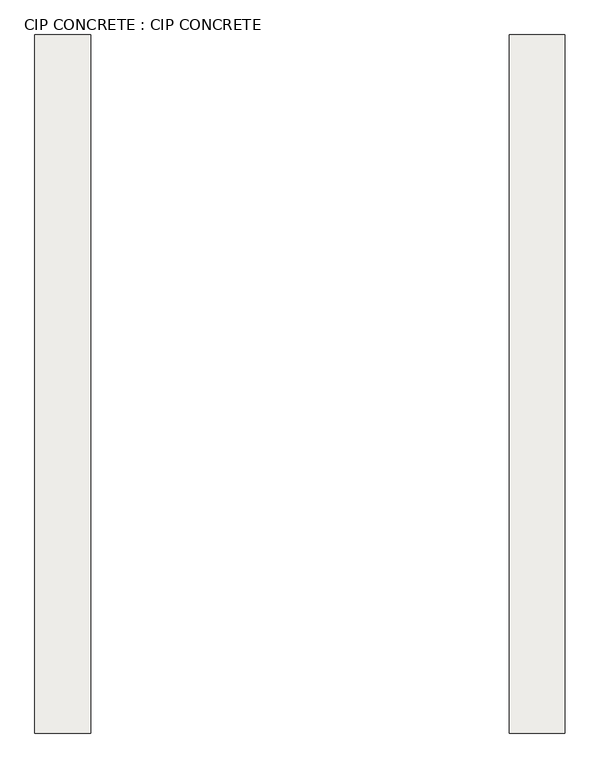
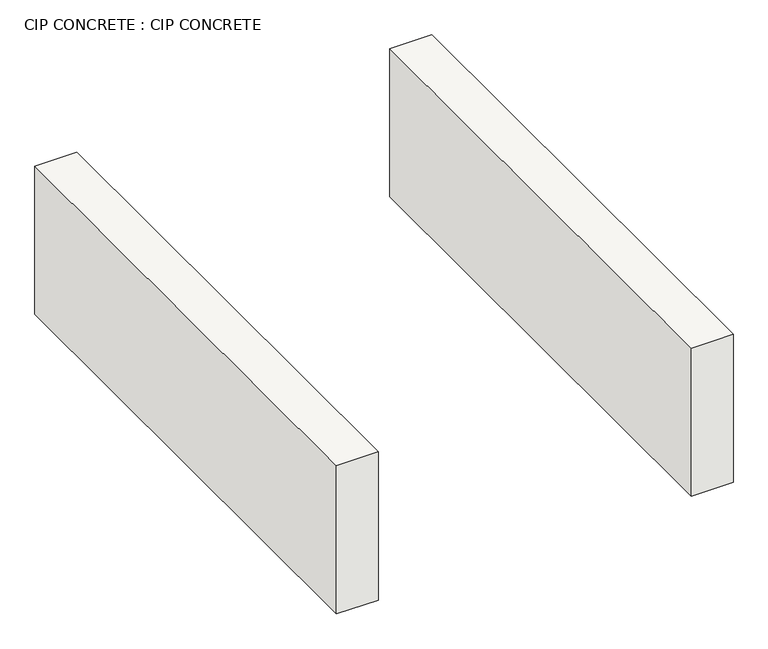
"""IFC4 building model written with IfcOpenShell, lengths in millimetres: slab geometry, CIP CONCRETE : CIP CONCRETE."""

from ifc_helpers import new_model, si_unit, frame, origin, place, context, project, spatial, polyline, outline, extrude, source, transform, mapped, element, save


def cip_concrete_cip_concrete_0247726a(model_context):
    return source(origin(), model_context, "Body", "SweptSolid", [
        extrude(outline(polyline([(14020.0, 38279.5208589), (14020.0, 33279.5208589), (13620.0, 33279.5208589), (13620.0, 38279.5208589), (14020.0, 38279.5208589)])), frame((0.0, 0.0, -1000.0), z_axis=(0.0, 0.0, 1.0), x_axis=(1.0, 0.0, 0.0)), (0.0, 0.0, 1.0), 1500.0),
        extrude(outline(polyline([(10620.0, 38279.5208589), (10620.0, 33279.5208589), (10220.0, 33279.5208589), (10220.0, 38279.5208589), (10620.0, 38279.5208589)])), frame((0.0, 0.0, -1000.0), z_axis=(0.0, 0.0, 1.0), x_axis=(1.0, 0.0, 0.0)), (0.0, 0.0, 1.0), 1500.0),
    ])


if __name__ == "__main__":
    model = new_model("IFC4")
    model_context = context("Model", 3, world=origin())
    ifc_project = project(units=[si_unit("LENGTHUNIT", "METRE", prefix="MILLI")], contexts=[model_context])
    site = spatial("IfcSite", under=ifc_project)
    building = spatial("IfcBuilding", under=site)
    placement = place(None, origin())
    cip_concrete_cip_concrete_shape = cip_concrete_cip_concrete_0247726a(model_context)
    element("IfcSlab", 1, ObjectType="CIP CONCRETE : CIP CONCRETE", at=placement, inside=building, context=model_context, shape_type="MappedRepresentation", body=[
        mapped(cip_concrete_cip_concrete_shape, transform((0.0, 0.0, 0.0), x_axis=(1.0, 0.0, 0.0), y_axis=(0.0, 1.0, 0.0), z_axis=(0.0, 0.0, 1.0))),
    ])
    save(model, "model.ifc")
